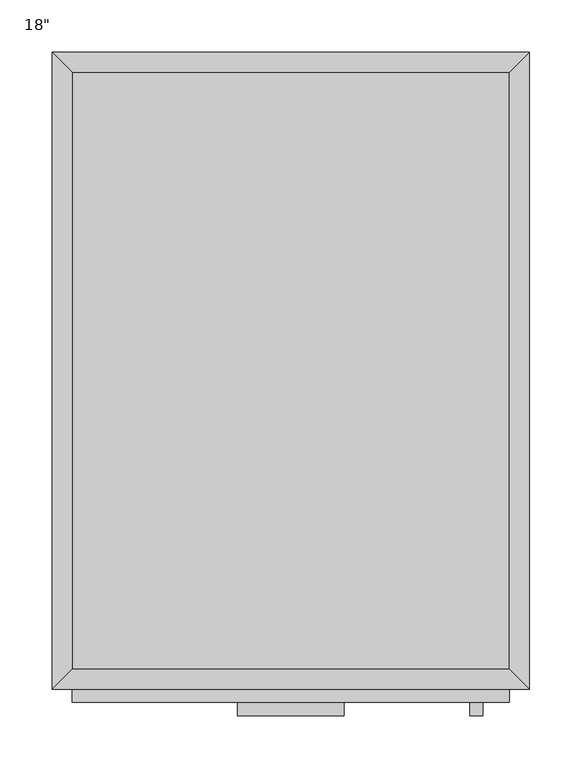
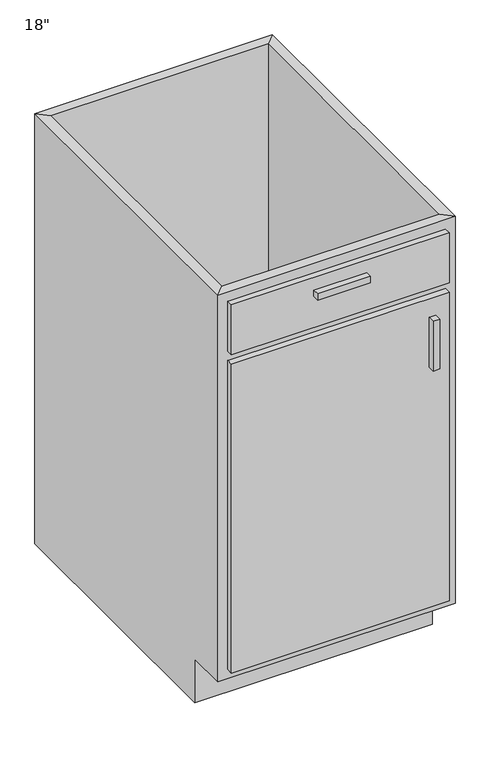
"""IFC4 building model written with IfcOpenShell, lengths in millimetres: furniture geometry."""

import ifcopenshell
import ifcopenshell.guid

model = None  # the IFC model being written
_history = None  # IfcOwnerHistory: only IFC2X3 demands one
_inside = {}  # id of a spatial element -> (the spatial element, [elements in it])
_under = {}  # id of a project, library or spatial element -> (it, [spatial elements below it])
_declared = {}  # id of a project -> (the project, [libraries it declares])
_typed = {}  # id of a type object -> (the type object, [elements of that type])
_made_of = {}  # id of a material, layer set ... -> (it, [elements and type objects made of it])


def new_model(schema):
    """Start an empty IFC model of exactly this schema.

    Asked for "IFC4X3", IfcOpenShell would pick the latest addendum, in which some entities
    have other attributes; the version numbers below select the first issue.
    IFC2X3 requires an IfcOwnerHistory on every rooted entity: one is made here for all.
    """
    global model, _history
    if schema == "IFC4X3":
        model = ifcopenshell.file(schema_version=(4, 3, 0, 0))
    else:
        model = ifcopenshell.file(schema=schema)
    _inside.clear()
    _under.clear()
    _declared.clear()
    _typed.clear()
    _made_of.clear()
    _history = None
    if model.schema == "IFC2X3":
        org = make("IfcOrganization", Name="unknown")
        user = make(
            "IfcPersonAndOrganization",
            ThePerson=make("IfcPerson", FamilyName="unknown"),
            TheOrganization=org,
        )
        app = make(
            "IfcApplication",
            ApplicationDeveloper=org,
            Version="unknown",
            ApplicationFullName="unknown",
            ApplicationIdentifier="unknown",
        )
        _history = make(
            "IfcOwnerHistory",
            OwningUser=user,
            OwningApplication=app,
            ChangeAction="ADDED",
            CreationDate=0,
        )
    return model


def make(cls, **values):
    """One entity of the class cls with the attributes given. An attribute that is None is left unset."""
    return model.create_entity(
        cls, **{name: value for name, value in values.items() if value is not None}
    )


def rooted(cls, **values):
    """An entity with a GlobalId (a new one), such as an element, a storey or a relation."""
    return make(cls, GlobalId=ifcopenshell.guid.new(), OwnerHistory=_history, **values)


def si_unit(unit_type, name, prefix=None):
    """IfcSIUnit, for example si_unit("LENGTHUNIT", "METRE", prefix="MILLI")."""
    return make("IfcSIUnit", UnitType=unit_type, Prefix=prefix, Name=name)


def assignment(units):
    """IfcUnitAssignment: the units of a project."""
    return None if units is None else make("IfcUnitAssignment", Units=units)


def point(xyz):
    """IfcCartesianPoint."""
    return None if xyz is None else make("IfcCartesianPoint", Coordinates=xyz)


def direction(xyz):
    """IfcDirection."""
    return None if xyz is None else make("IfcDirection", DirectionRatios=xyz)


def frame(location, z_axis=None, x_axis=None):
    """IfcAxis2Placement3D, a coordinate frame: its origin and axes. An axis left out is left unset."""
    return make(
        "IfcAxis2Placement3D",
        Location=point(location),
        Axis=direction(z_axis),
        RefDirection=direction(x_axis),
    )


def origin():
    """The frame at (0, 0, 0) with its axes left unset."""
    return frame((0.0, 0.0, 0.0))


def place(relative_to, where):
    """IfcLocalPlacement: puts the frame where relative to a parent placement (None: the world)."""
    return make(
        "IfcLocalPlacement", PlacementRelTo=relative_to, RelativePlacement=where
    )


def context(
    kind, dimensions, precision=None, world=None, true_north=None, identifier=None
):
    """IfcGeometricRepresentationContext, for example the 3D "Model" context."""
    return make(
        "IfcGeometricRepresentationContext",
        ContextIdentifier=identifier,
        ContextType=kind,
        CoordinateSpaceDimension=dimensions,
        Precision=precision,
        WorldCoordinateSystem=world,
        TrueNorth=true_north,
    )


def project(units=None, contexts=None):
    """IfcProject with its units and contexts."""
    return rooted(
        "IfcProject",
        Name="project",
        RepresentationContexts=contexts,
        UnitsInContext=assignment(units),
    )


def spatial(cls, under=None, at=None, **own):
    """A site, building, storey or space (cls), placed at a placement, below another one or the project."""
    s = rooted(cls, ObjectPlacement=at, **own)
    if under is not None:
        _under.setdefault(under.id(), (under, []))[1].append(s)
    return s


def polyline(points):
    """IfcPolyline through the points."""
    return make("IfcPolyline", Points=[point(p) for p in points])


def outline(outer, holes=None, kind="AREA"):
    """IfcArbitraryClosedProfileDef: a profile drawn as a closed curve; with holes, ...WithVoids."""
    if holes is None:
        return make("IfcArbitraryClosedProfileDef", ProfileType=kind, OuterCurve=outer)
    return make(
        "IfcArbitraryProfileDefWithVoids",
        ProfileType=kind,
        OuterCurve=outer,
        InnerCurves=holes,
    )


def extrude(swept, where, along, depth):
    """IfcExtrudedAreaSolid: the profile swept, set in the frame where, extruded along a direction by depth."""
    return make(
        "IfcExtrudedAreaSolid",
        SweptArea=swept,
        Position=where,
        ExtrudedDirection=direction(along),
        Depth=depth,
    )


def faces_of(points, faces, orient=None, outer=None):
    """IfcFace entities. A face is a list of loops; a loop is a list of indices into points, from 0.

    orient and outer hold one flag for each loop. By default every Orientation is true, the
    first loop of a face is its IfcFaceOuterBound and the others are IfcFaceBound.
    """
    made = []
    for i, loops in enumerate(faces):
        bounds = []
        for j, loop in enumerate(loops):
            is_outer = j == 0 if outer is None else outer[i][j]
            bounds.append(
                make(
                    "IfcFaceOuterBound" if is_outer else "IfcFaceBound",
                    Bound=make("IfcPolyLoop", Polygon=[points[k] for k in loop]),
                    Orientation=True if orient is None else orient[i][j],
                )
            )
        made.append(make("IfcFace", Bounds=bounds))
    return made


def faceted_brep(points, faces, orient=None, outer=None, voids=None):
    """IfcFacetedBrep: a solid bounded by flat faces; with voids (closed shells), ...WithVoids."""
    shared = [point(p) for p in points]
    hull = make("IfcClosedShell", CfsFaces=faces_of(shared, faces, orient, outer))
    if voids is None:
        return make("IfcFacetedBrep", Outer=hull)
    return make(
        "IfcFacetedBrepWithVoids",
        Outer=hull,
        Voids=[
            make(cls, CfsFaces=faces_of(shared, fs, o, b)) for cls, fs, o, b in voids
        ],
    )


def shape(context_of_items, identifier, shape_type, items):
    """IfcShapeRepresentation: the items that make up one representation, for example the "Body"."""
    return make(
        "IfcShapeRepresentation",
        ContextOfItems=context_of_items,
        RepresentationIdentifier=identifier,
        RepresentationType=shape_type,
        Items=items,
    )


def source(mapping_origin, context_of_items, identifier, shape_type, items):
    """IfcRepresentationMap: a shape defined once, which mapped items show again and again."""
    return make(
        "IfcRepresentationMap",
        MappingOrigin=mapping_origin,
        MappedRepresentation=shape(context_of_items, identifier, shape_type, items),
    )


def transform(
    local_origin,
    x_axis=None,
    y_axis=None,
    z_axis=None,
    scale=None,
    scale2=None,
    scale3=None,
    uniform=True,
):
    """IfcCartesianTransformationOperator3D, or its non-uniform kind. x_axis, y_axis, z_axis: its Axis1, 2, 3."""
    if uniform:
        return make(
            "IfcCartesianTransformationOperator3D",
            Axis1=direction(x_axis),
            Axis2=direction(y_axis),
            LocalOrigin=point(local_origin),
            Scale=scale,
            Axis3=direction(z_axis),
        )
    return make(
        "IfcCartesianTransformationOperator3DnonUniform",
        Axis1=direction(x_axis),
        Axis2=direction(y_axis),
        LocalOrigin=point(local_origin),
        Scale=scale,
        Axis3=direction(z_axis),
        Scale2=scale2,
        Scale3=scale3,
    )


def mapped(mapping_source, mapping_target):
    """IfcMappedItem: shows the shape of a source again, moved by a transform."""
    return make(
        "IfcMappedItem", MappingSource=mapping_source, MappingTarget=mapping_target
    )


def made_of(thing, what):
    """Note that an element or type object is made of a material, layer set ...; save() writes the relation."""
    if what is not None:
        _made_of.setdefault(what.id(), (what, []))[1].append(thing)
    return thing


def element(
    cls,
    number,
    at=None,
    inside=None,
    cuts=None,
    type_object=None,
    material=None,
    context=None,
    identifier="Body",
    shape_type=None,
    held_by="IfcProductDefinitionShape",
    body=None,
    shapes=None,
    **own,
):
    """One element of the class cls, such as IfcWall. Its Tag is "e" and its number.

    at: its placement. inside: the storey or other place that contains it. cuts: it is an
    opening in that element (IfcRelVoidsElement). A single representation is given by context,
    identifier, shape_type and body (its items); several are given by shapes. held_by: the class
    of the entity that holds the representations. save() writes the other relations.
    """
    e = rooted(cls, Tag="e%d" % number, ObjectPlacement=at, **own)
    if body is not None:
        shapes = [shape(context, identifier, shape_type, body)]
    if shapes is not None:
        e.Representation = make(held_by, Representations=shapes)
    if inside is not None:
        _inside.setdefault(inside.id(), (inside, []))[1].append(e)
    if cuts is not None:
        rooted(
            "IfcRelVoidsElement", RelatingBuildingElement=cuts, RelatedOpeningElement=e
        )
    if type_object is not None:
        _typed.setdefault(type_object.id(), (type_object, []))[1].append(e)
    return made_of(e, material)


def aggregate(whole, parts):
    """IfcRelAggregates: a whole, such as a stair, and the parts it consists of."""
    return rooted("IfcRelAggregates", RelatingObject=whole, RelatedObjects=parts)


def save(model, path):
    """Write the relations noted so far, then the file.

    IfcRelAggregates (storeys below a building ...), IfcRelContainedInSpatialStructure (elements
    in a storey), IfcRelDefinesByType, IfcRelAssociatesMaterial and IfcRelDeclares: one each for
    every whole, place, type object, material and project.
    """
    for whole, parts in _under.values():
        aggregate(whole, parts)
    for where, things in _inside.values():
        rooted(
            "IfcRelContainedInSpatialStructure",
            RelatedElements=things,
            RelatingStructure=where,
        )
    for kind, things in _typed.values():
        rooted("IfcRelDefinesByType", RelatedObjects=things, RelatingType=kind)
    for what, things in _made_of.values():
        rooted("IfcRelAssociatesMaterial", RelatedObjects=things, RelatingMaterial=what)
    for by, libraries in _declared.values():
        rooted("IfcRelDeclares", RelatingContext=by, RelatedDefinitions=libraries)
    model.write(path)


def furniture_6ace90bf(model_context):
    return source(origin(), model_context, "Body", "SolidModel", [
        faceted_brep([(228.2877049, -590.55, 876.3), (228.2877049, -590.55, 88.9), (-190.8122951, -590.55, 88.9), (-190.8122951, -590.55, 876.3), (-209.8622951, -609.6, 876.3), (247.3377049, -609.6, 876.3), (-209.8622951, -609.6, 88.9), (247.3377049, -609.6, 88.9), (-190.8122951, -533.4, 88.9), (-190.8122951, -19.05, 88.9), (-190.8122951, -19.05, 876.3), (-209.8622951, 0.0, 876.3), (-209.8622951, 0.0, 0.0), (-209.8622951, -533.4, 0.0), (-209.8622951, -533.4, 88.9), (228.2877049, -19.05, 88.9), (228.2877049, -19.05, 876.3), (247.3377049, 0.0, 876.3), (247.3377049, 0.0, 0.0), (228.2877049, -533.4, 88.9), (247.3377049, -533.4, 88.9), (247.3377049, -533.4, 0.0)], [[[0, 1, 2, 3]], [[0, 3, 4, 5]], [[5, 4, 6, 7]], [[2, 1, 7, 6]], [[3, 2, 8, 9, 10]], [[4, 3, 10, 11]], [[6, 4, 11, 12, 13, 14]], [[2, 6, 14, 8]], [[10, 9, 15, 16]], [[11, 10, 16, 17]], [[12, 11, 17, 18]], [[1, 0, 16, 15, 19]], [[0, 5, 17, 16]], [[5, 7, 20, 21, 18, 17]], [[7, 1, 19, 20]], [[8, 19, 15, 9]], [[18, 21, 13, 12]], [[13, 21, 20, 19, 8, 14]]]),
        extrude(outline(polyline([(202.8877049, -635.0), (190.1877049, -635.0), (190.1877049, -622.3), (202.8877049, -622.3), (202.8877049, -635.0)])), frame((0.0, 0.0, 596.9), z_axis=(0.0, 0.0, 1.0), x_axis=(1.0, 0.0, 0.0)), (0.0, 0.0, 1.0), 101.6),
        extrude(outline(polyline([(69.5377049, -635.0), (-32.0622951, -635.0), (-32.0622951, -622.3), (69.5377049, -622.3), (69.5377049, -635.0)])), frame((0.0, 0.0, 819.15), z_axis=(0.0, 0.0, 1.0), x_axis=(1.0, 0.0, 0.0)), (0.0, 0.0, 1.0), 12.7),
        extrude(outline(polyline([(228.2877049, -622.3), (-190.8122951, -622.3), (-190.8122951, -609.6), (228.2877049, -609.6), (228.2877049, -622.3)])), frame((0.0, 0.0, 107.95), z_axis=(0.0, 0.0, 1.0), x_axis=(1.0, 0.0, 0.0)), (0.0, 0.0, 1.0), 628.65),
        extrude(outline(polyline([(228.2877049, -622.3), (-190.8122951, -622.3), (-190.8122951, -609.6), (228.2877049, -609.6), (228.2877049, -622.3)])), frame((0.0, 0.0, 755.65), z_axis=(0.0, 0.0, 1.0), x_axis=(1.0, 0.0, 0.0)), (0.0, 0.0, 1.0), 101.6),
        extrude(outline(polyline([(228.2877049, -19.05), (228.2877049, -590.55), (-190.8122951, -590.55), (-190.8122951, -19.05), (228.2877049, -19.05)])), frame((0.0, 0.0, 88.9), z_axis=(0.0, 0.0, 1.0), x_axis=(1.0, 0.0, 0.0)), (0.0, 0.0, 1.0), 19.05),
    ])


if __name__ == "__main__":
    model = new_model("IFC4")
    model_context = context("Model", 3, world=origin())
    ifc_project = project(units=[si_unit("LENGTHUNIT", "METRE", prefix="MILLI")], contexts=[model_context])
    site = spatial("IfcSite", under=ifc_project)
    building = spatial("IfcBuilding", under=site)
    placement = place(None, origin())
    furniture_shape = furniture_6ace90bf(model_context)
    element("IfcFurniture", 1, ObjectType="Base Cabinet-Single Door & Drawer : 18\"", at=placement, inside=building, context=model_context, shape_type="MappedRepresentation", body=[
        mapped(furniture_shape, transform((0.0, 0.0, 0.0), x_axis=(1.0, 0.0, 0.0), y_axis=(0.0, 1.0, 0.0), z_axis=(0.0, 0.0, 1.0))),
    ])
    save(model, "model.ifc")

# Revit data of these elements
# Type "Base Cabinet-Single Door & Drawer : 18\""
#   COBie.Type.CreatedBy = "doug.wood@us.ibm.com"
#   COBie.Type.CreatedOn = "2016-04-14T02:14:45"
#   COBie.Type.Name = "Casework_Base Cabinet-Single Door & Drawer_18\""
#   COBie.Type.Category = "23-40 35 17 47 11 : Kitchen Casework"
#   COBie.Type.Description = "Base Cabinet-Single Door & Drawer_18\""
#   COBie.Type.Manufacturer = ""
#   COBie.Type.ModelNumber = ""
#   Assembly Code = "C1030410"
#   COBie.Type.ReplacementCost = 0
#   Depth = 2' - 0"
#   Height = 2' - 10 1/2"
#   Toe Depth = 0' - 3"
#   Toe Height = 0' - 3 1/2"
#   Width = 1' - 6"
#   COBie.Type = no
#   Cabinet Material = none
#   Drawer Material = none
#   Handle Material = Cabinets - Handles
# Element 1 (IfcFurniture, "Base Cabinet-Single Door & Drawer : 18\"")
#   Materials on its faces: "Cabinets", "Cabinets - Handles"
# Materials
#   "Cabinets - Handles": class "Metal", colour RGB 57 57 57, transparency 0
#   "Cabinets": class "Miscellaneous", colour RGB 249 249 249, transparency 0
